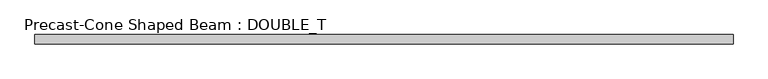
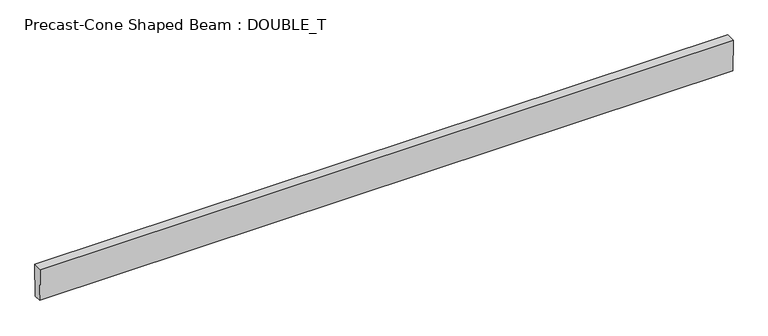
"""IFC4 building model written with IfcOpenShell, lengths in millimetres: beam geometry, Precast-Cone Shaped Beam : DOUBLE_T."""

from ifc_helpers import new_model, si_unit, frame, origin, place, context, project, spatial, polyline, outline, extrude, source, transform, mapped, element, save


def precast_cone_shaped_beam_double_t_5ff23cd5(model_context):
    return source(origin(), model_context, "Body", "SweptSolid", [
        extrude(outline(polyline([(-50.8, -228.6), (-63.5, 228.6), (63.5, 228.6), (50.8, -228.6), (-50.8, -228.6)])), frame((-4660.9, 0.0, 0.0), z_axis=(1.0, 0.0, 0.0), x_axis=(0.0, 1.0, 0.0)), (0.0, 0.0, 1.0), 9601.2),
    ])


if __name__ == "__main__":
    model = new_model("IFC4")
    model_context = context("Model", 3, world=origin())
    ifc_project = project(units=[si_unit("LENGTHUNIT", "METRE", prefix="MILLI")], contexts=[model_context])
    site = spatial("IfcSite", under=ifc_project)
    building = spatial("IfcBuilding", under=site)
    placement = place(None, origin())
    precast_cone_shaped_beam_double_t_shape = precast_cone_shaped_beam_double_t_5ff23cd5(model_context)
    element("IfcBeam", 1, ObjectType="Precast-Cone Shaped Beam : DOUBLE_T", at=placement, inside=building, context=model_context, shape_type="MappedRepresentation", body=[
        mapped(precast_cone_shaped_beam_double_t_shape, transform((0.0, 0.0, 0.0), x_axis=(1.0, 0.0, 0.0), y_axis=(0.0, 1.0, 0.0), z_axis=(0.0, 0.0, 1.0))),
    ])
    save(model, "model.ifc")

# Revit data of these elements
# Type "Precast-Cone Shaped Beam : DOUBLE_T"
#   Top Width = 0' - 5"
#   Tie Rod Weight [instance default] = 30
#   Tie Rod W [instance default] = 0.0660938 kip
#   Single Rebar Weight [instance default] = 50
#   Single Rebar W [instance default] = 0.110156 kip
#   Rebar Grids Weight [instance default] = 100
#   Rebar Grids W [instance default] = 0.220313 kip
#   Depth = 1' - 6"
#   Bottom Width = 0' - 4"
#   Length [instance default] = 5' - 0"
#   Structural Material [instance default] = Concrete, Precast
#   Assembly Code = ""
# Element 1 (IfcBeam, "Precast-Cone Shaped Beam : DOUBLE_T")
#   Length = 31' - 7"
#   Structural Material = Concrete - Precast Concrete - Normal Weight Concrete - 5 ksi
#   Materials on its faces: "Concrete - Precast Concrete - Normal Weight Concrete - 5 ksi"
# Materials
#   "Concrete, Precast": class "Concrete", colour RGB 198 187 187, transparency 0, Description = "Precast concrete", Cost = 0
#   "Concrete - Precast Concrete - Normal Weight Concrete - 5 ksi": class "Concrete", colour RGB 198 187 187, transparency 0, Cost = 0
